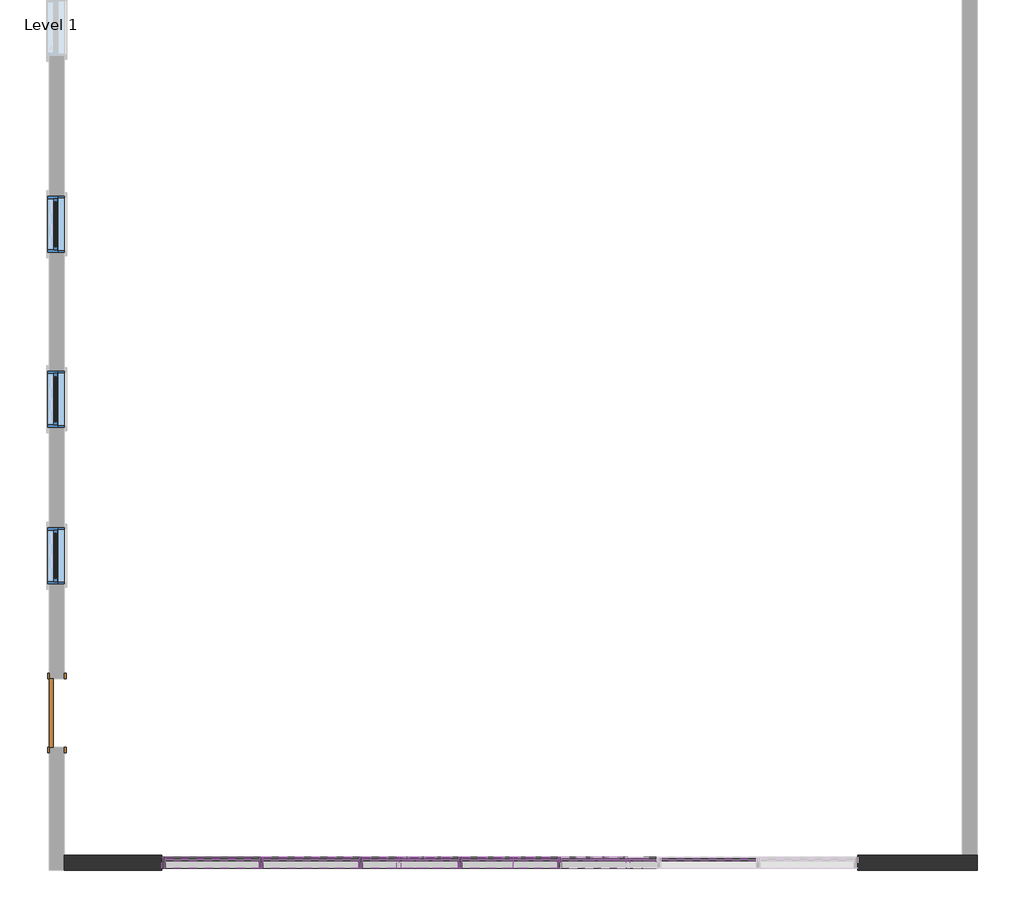
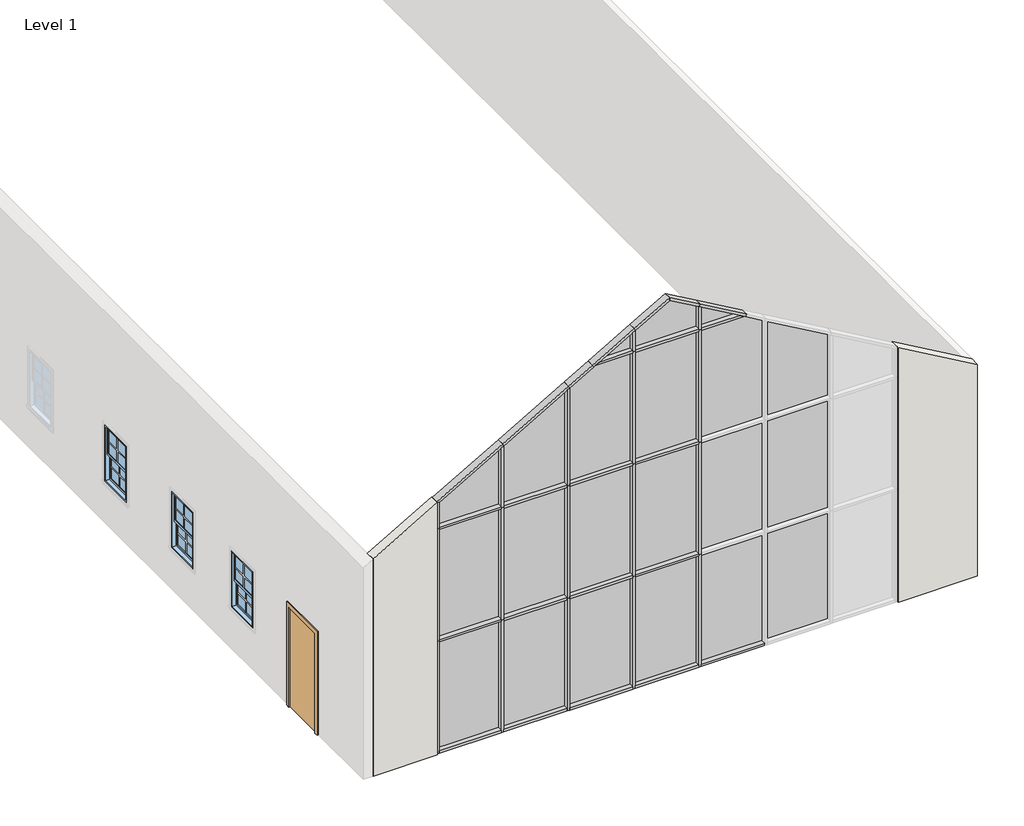
# One storey, part 1 of 2: 40 members, 21 plates, 3 windows, 1 door, 1 wall.
"""IFC4 building model written with IfcOpenShell, lengths in millimetres."""

import ifcopenshell
import ifcopenshell.guid

model = None  # the IFC model being written
_history = None  # IfcOwnerHistory: only IFC2X3 demands one
_inside = {}  # id of a spatial element -> (the spatial element, [elements in it])
_under = {}  # id of a project, library or spatial element -> (it, [spatial elements below it])
_declared = {}  # id of a project -> (the project, [libraries it declares])
_typed = {}  # id of a type object -> (the type object, [elements of that type])
_made_of = {}  # id of a material, layer set ... -> (it, [elements and type objects made of it])


def new_model(schema):
    """Start an empty IFC model of exactly this schema.

    Asked for "IFC4X3", IfcOpenShell would pick the latest addendum, in which some entities
    have other attributes; the version numbers below select the first issue.
    IFC2X3 requires an IfcOwnerHistory on every rooted entity: one is made here for all.
    """
    global model, _history
    if schema == "IFC4X3":
        model = ifcopenshell.file(schema_version=(4, 3, 0, 0))
    else:
        model = ifcopenshell.file(schema=schema)
    _inside.clear()
    _under.clear()
    _declared.clear()
    _typed.clear()
    _made_of.clear()
    _history = None
    if model.schema == "IFC2X3":
        org = make("IfcOrganization", Name="unknown")
        user = make(
            "IfcPersonAndOrganization",
            ThePerson=make("IfcPerson", FamilyName="unknown"),
            TheOrganization=org,
        )
        app = make(
            "IfcApplication",
            ApplicationDeveloper=org,
            Version="unknown",
            ApplicationFullName="unknown",
            ApplicationIdentifier="unknown",
        )
        _history = make(
            "IfcOwnerHistory",
            OwningUser=user,
            OwningApplication=app,
            ChangeAction="ADDED",
            CreationDate=0,
        )
    return model


def make(cls, **values):
    """One entity of the class cls with the attributes given. An attribute that is None is left unset."""
    return model.create_entity(
        cls, **{name: value for name, value in values.items() if value is not None}
    )


def rooted(cls, **values):
    """An entity with a GlobalId (a new one), such as an element, a storey or a relation."""
    return make(cls, GlobalId=ifcopenshell.guid.new(), OwnerHistory=_history, **values)


def si_unit(unit_type, name, prefix=None):
    """IfcSIUnit, for example si_unit("LENGTHUNIT", "METRE", prefix="MILLI")."""
    return make("IfcSIUnit", UnitType=unit_type, Prefix=prefix, Name=name)


def assignment(units):
    """IfcUnitAssignment: the units of a project."""
    return None if units is None else make("IfcUnitAssignment", Units=units)


def point(xyz):
    """IfcCartesianPoint."""
    return None if xyz is None else make("IfcCartesianPoint", Coordinates=xyz)


def direction(xyz):
    """IfcDirection."""
    return None if xyz is None else make("IfcDirection", DirectionRatios=xyz)


def frame(location, z_axis=None, x_axis=None):
    """IfcAxis2Placement3D, a coordinate frame: its origin and axes. An axis left out is left unset."""
    return make(
        "IfcAxis2Placement3D",
        Location=point(location),
        Axis=direction(z_axis),
        RefDirection=direction(x_axis),
    )


def origin():
    """The frame at (0, 0, 0) with its axes left unset."""
    return frame((0.0, 0.0, 0.0))


def origin_with_axes():
    """The frame at (0, 0, 0) with the z axis (0, 0, 1) and the x axis (1, 0, 0) written out."""
    return frame((0.0, 0.0, 0.0), z_axis=(0.0, 0.0, 1.0), x_axis=(1.0, 0.0, 0.0))


def place(relative_to, where):
    """IfcLocalPlacement: puts the frame where relative to a parent placement (None: the world)."""
    return make(
        "IfcLocalPlacement", PlacementRelTo=relative_to, RelativePlacement=where
    )


def context(
    kind, dimensions, precision=None, world=None, true_north=None, identifier=None
):
    """IfcGeometricRepresentationContext, for example the 3D "Model" context."""
    return make(
        "IfcGeometricRepresentationContext",
        ContextIdentifier=identifier,
        ContextType=kind,
        CoordinateSpaceDimension=dimensions,
        Precision=precision,
        WorldCoordinateSystem=world,
        TrueNorth=true_north,
    )


def project(units=None, contexts=None):
    """IfcProject with its units and contexts."""
    return rooted(
        "IfcProject",
        Name="project",
        RepresentationContexts=contexts,
        UnitsInContext=assignment(units),
    )


def spatial(cls, under=None, at=None, **own):
    """A site, building, storey or space (cls), placed at a placement, below another one or the project."""
    s = rooted(cls, ObjectPlacement=at, **own)
    if under is not None:
        _under.setdefault(under.id(), (under, []))[1].append(s)
    return s


def polyline(points):
    """IfcPolyline through the points."""
    return make("IfcPolyline", Points=[point(p) for p in points])


def outline(outer, holes=None, kind="AREA"):
    """IfcArbitraryClosedProfileDef: a profile drawn as a closed curve; with holes, ...WithVoids."""
    if holes is None:
        return make("IfcArbitraryClosedProfileDef", ProfileType=kind, OuterCurve=outer)
    return make(
        "IfcArbitraryProfileDefWithVoids",
        ProfileType=kind,
        OuterCurve=outer,
        InnerCurves=holes,
    )


def extrude(swept, where, along, depth):
    """IfcExtrudedAreaSolid: the profile swept, set in the frame where, extruded along a direction by depth."""
    return make(
        "IfcExtrudedAreaSolid",
        SweptArea=swept,
        Position=where,
        ExtrudedDirection=direction(along),
        Depth=depth,
    )


def faces_of(points, faces, orient=None, outer=None):
    """IfcFace entities. A face is a list of loops; a loop is a list of indices into points, from 0.

    orient and outer hold one flag for each loop. By default every Orientation is true, the
    first loop of a face is its IfcFaceOuterBound and the others are IfcFaceBound.
    """
    made = []
    for i, loops in enumerate(faces):
        bounds = []
        for j, loop in enumerate(loops):
            is_outer = j == 0 if outer is None else outer[i][j]
            bounds.append(
                make(
                    "IfcFaceOuterBound" if is_outer else "IfcFaceBound",
                    Bound=make("IfcPolyLoop", Polygon=[points[k] for k in loop]),
                    Orientation=True if orient is None else orient[i][j],
                )
            )
        made.append(make("IfcFace", Bounds=bounds))
    return made


def faceted_brep(points, faces, orient=None, outer=None, voids=None):
    """IfcFacetedBrep: a solid bounded by flat faces; with voids (closed shells), ...WithVoids."""
    shared = [point(p) for p in points]
    hull = make("IfcClosedShell", CfsFaces=faces_of(shared, faces, orient, outer))
    if voids is None:
        return make("IfcFacetedBrep", Outer=hull)
    return make(
        "IfcFacetedBrepWithVoids",
        Outer=hull,
        Voids=[
            make(cls, CfsFaces=faces_of(shared, fs, o, b)) for cls, fs, o, b in voids
        ],
    )


def shape(context_of_items, identifier, shape_type, items):
    """IfcShapeRepresentation: the items that make up one representation, for example the "Body"."""
    return make(
        "IfcShapeRepresentation",
        ContextOfItems=context_of_items,
        RepresentationIdentifier=identifier,
        RepresentationType=shape_type,
        Items=items,
    )


def source(mapping_origin, context_of_items, identifier, shape_type, items):
    """IfcRepresentationMap: a shape defined once, which mapped items show again and again."""
    return make(
        "IfcRepresentationMap",
        MappingOrigin=mapping_origin,
        MappedRepresentation=shape(context_of_items, identifier, shape_type, items),
    )


def transform(
    local_origin,
    x_axis=None,
    y_axis=None,
    z_axis=None,
    scale=None,
    scale2=None,
    scale3=None,
    uniform=True,
):
    """IfcCartesianTransformationOperator3D, or its non-uniform kind. x_axis, y_axis, z_axis: its Axis1, 2, 3."""
    if uniform:
        return make(
            "IfcCartesianTransformationOperator3D",
            Axis1=direction(x_axis),
            Axis2=direction(y_axis),
            LocalOrigin=point(local_origin),
            Scale=scale,
            Axis3=direction(z_axis),
        )
    return make(
        "IfcCartesianTransformationOperator3DnonUniform",
        Axis1=direction(x_axis),
        Axis2=direction(y_axis),
        LocalOrigin=point(local_origin),
        Scale=scale,
        Axis3=direction(z_axis),
        Scale2=scale2,
        Scale3=scale3,
    )


def mapped(mapping_source, mapping_target):
    """IfcMappedItem: shows the shape of a source again, moved by a transform."""
    return make(
        "IfcMappedItem", MappingSource=mapping_source, MappingTarget=mapping_target
    )


def made_of(thing, what):
    """Note that an element or type object is made of a material, layer set ...; save() writes the relation."""
    if what is not None:
        _made_of.setdefault(what.id(), (what, []))[1].append(thing)
    return thing


def element(
    cls,
    number,
    at=None,
    inside=None,
    cuts=None,
    type_object=None,
    material=None,
    context=None,
    identifier="Body",
    shape_type=None,
    held_by="IfcProductDefinitionShape",
    body=None,
    shapes=None,
    **own,
):
    """One element of the class cls, such as IfcWall. Its Tag is "e" and its number.

    at: its placement. inside: the storey or other place that contains it. cuts: it is an
    opening in that element (IfcRelVoidsElement). A single representation is given by context,
    identifier, shape_type and body (its items); several are given by shapes. held_by: the class
    of the entity that holds the representations. save() writes the other relations.
    """
    e = rooted(cls, Tag="e%d" % number, ObjectPlacement=at, **own)
    if body is not None:
        shapes = [shape(context, identifier, shape_type, body)]
    if shapes is not None:
        e.Representation = make(held_by, Representations=shapes)
    if inside is not None:
        _inside.setdefault(inside.id(), (inside, []))[1].append(e)
    if cuts is not None:
        rooted(
            "IfcRelVoidsElement", RelatingBuildingElement=cuts, RelatedOpeningElement=e
        )
    if type_object is not None:
        _typed.setdefault(type_object.id(), (type_object, []))[1].append(e)
    return made_of(e, material)


def aggregate(whole, parts):
    """IfcRelAggregates: a whole, such as a stair, and the parts it consists of."""
    return rooted("IfcRelAggregates", RelatingObject=whole, RelatedObjects=parts)


def save(model, path):
    """Write the relations noted so far, then the file.

    IfcRelAggregates (storeys below a building ...), IfcRelContainedInSpatialStructure (elements
    in a storey), IfcRelDefinesByType, IfcRelAssociatesMaterial and IfcRelDeclares: one each for
    every whole, place, type object, material and project.
    """
    for whole, parts in _under.values():
        aggregate(whole, parts)
    for where, things in _inside.values():
        rooted(
            "IfcRelContainedInSpatialStructure",
            RelatedElements=things,
            RelatingStructure=where,
        )
    for kind, things in _typed.values():
        rooted("IfcRelDefinesByType", RelatedObjects=things, RelatingType=kind)
    for what, things in _made_of.values():
        rooted("IfcRelAssociatesMaterial", RelatedObjects=things, RelatingMaterial=what)
    for by, libraries in _declared.values():
        rooted("IfcRelDeclares", RelatingContext=by, RelatedDefinitions=libraries)
    model.write(path)


def m_single_flush_0915_x_2134mm_6a9e8738(model_context):
    return source(origin(), model_context, "Body", "SweptSolid", [
        extrude(outline(polyline([(2210.0, -533.5), (0.0, -533.5), (0.0, -457.5), (2134.0, -457.5), (2134.0, 457.5), (0.0, 457.5), (0.0, 533.5), (2210.0, 533.5), (2210.0, -533.5)])), frame((0.0, 100.0, 0.0), z_axis=(0.0, 1.0, 0.0), x_axis=(0.0, 0.0, 1.0)), (0.0, 0.0, 1.0), 25.0),
        extrude(outline(polyline([(2210.0, 533.5), (2210.0, -533.5), (0.0, -533.5), (0.0, -457.5), (2134.0, -457.5), (2134.0, 457.5), (0.0, 457.5), (0.0, 533.5), (2210.0, 533.5)])), frame((0.0, -125.0, 0.0), z_axis=(0.0, 1.0, 0.0), x_axis=(0.0, 0.0, 1.0)), (0.0, 0.0, 1.0), 25.0),
        extrude(outline(polyline([(457.5, 49.0), (-457.5, 49.0), (-457.5, 100.0), (457.5, 100.0), (457.5, 49.0)])), origin_with_axes(), (0.0, 0.0, 1.0), 2134.0),
    ])


def rectangular_mullion_50mm_x_150mm_302a0cfa(model_context):
    return source(origin(), model_context, "Body", "SweptSolid", [
        extrude(outline(polyline([(0.0, 75.0), (0.0, -75.0), (-50.0, -75.0), (-50.0, 75.0), (0.0, 75.0)])), frame((0.0, 0.0, -1253.5714288), z_axis=(0.0, 0.0, 1.0), x_axis=(1.0, 0.0, 0.0)), (0.0, 0.0, 1.0), 1253.5714288),
    ])


def rectangular_mullion_50mm_x_150mm_11a5ee59(model_context):
    return source(origin(), model_context, "Body", "SweptSolid", [
        extrude(outline(polyline([(0.0, 75.0), (0.0, -75.0), (-50.0, -75.0), (-50.0, 75.0), (0.0, 75.0)])), frame((0.0, 0.0, -1278.5714285), z_axis=(0.0, 0.0, 1.0), x_axis=(1.0, 0.0, 0.0)), (0.0, 0.0, 1.0), 1278.5714285),
    ])


def rectangular_mullion_50mm_x_150mm_46426fc7(model_context):
    return source(origin(), model_context, "Body", "SweptSolid", [
        extrude(outline(polyline([(25.0, 75.0), (25.0, -75.0), (-25.0, -75.0), (-25.0, 75.0), (25.0, 75.0)])), frame((0.0, 0.0, -1253.5714288), z_axis=(0.0, 0.0, 1.0), x_axis=(1.0, 0.0, 0.0)), (0.0, 0.0, 1.0), 1253.5714288),
    ])


def rectangular_mullion_50mm_x_150mm_f38f42f6(model_context):
    return source(origin(), model_context, "Body", "SweptSolid", [
        extrude(outline(polyline([(25.0, 75.0), (25.0, -75.0), (-25.0, -75.0), (-25.0, 75.0), (25.0, 75.0)])), frame((0.0, 0.0, -1278.5714285), z_axis=(0.0, 0.0, 1.0), x_axis=(1.0, 0.0, 0.0)), (0.0, 0.0, 1.0), 1278.5714285),
    ])


def rectangular_mullion_50mm_x_150mm_6225e4e3(model_context):
    return source(origin(), model_context, "Body", "SweptSolid", [
        extrude(outline(polyline([(25.0, 75.0), (25.0, -75.0), (-25.0, -75.0), (-25.0, 75.0), (25.0, 75.0)])), frame((0.0, 0.0, -2400.0), z_axis=(0.0, 0.0, 1.0), x_axis=(1.0, 0.0, 0.0)), (0.0, 0.0, 1.0), 2400.0),
    ])


def rectangular_mullion_50mm_x_150mm_662c37b1(model_context):
    return source(origin(), model_context, "Body", "SweptSolid", [
        extrude(outline(polyline([(0.0, 75.0), (0.0, -75.0), (-50.0, -75.0), (-50.0, 75.0), (0.0, 75.0)])), frame((0.0, 0.0, -2400.0), z_axis=(0.0, 0.0, 1.0), x_axis=(1.0, 0.0, 0.0)), (0.0, 0.0, 1.0), 2400.0),
    ])


def rectangular_mullion_50mm_x_150mm_ac9de802(model_context):
    return source(origin(), model_context, "Body", "SweptSolid", [
        extrude(outline(polyline([(0.0, 25.0), (0.0, -25.0), (-761.4529717, -25.0), (-674.8504313, 25.0), (0.0, 25.0)])), frame((0.0, -75.0, 0.0), z_axis=(0.0, 1.0, 0.0), x_axis=(0.0, 0.0, 1.0)), (0.0, 0.0, 1.0), 150.0),
    ])


def rectangular_mullion_50mm_x_150mm_f9b92fbf(model_context):
    return source(origin(), model_context, "Body", "SweptSolid", [
        extrude(outline(polyline([(-143.3012702, 25.0), (-56.6987298, -25.0), (-918.1517015, -25.0), (-918.1517015, 25.0), (-143.3012702, 25.0)])), frame((0.0, -75.0, 0.0), z_axis=(0.0, 1.0, 0.0), x_axis=(0.0, 0.0, 1.0)), (0.0, 0.0, 1.0), 150.0),
    ])


def rectangular_mullion_50mm_x_150mm_ea3fe943(model_context):
    return source(origin(), model_context, "Body", "SweptSolid", [
        extrude(outline(polyline([(0.0, 25.0), (0.0, -25.0), (-1280.5229345, -25.0), (-1309.3904479, 25.0), (0.0, 25.0)])), frame((0.0, -75.0, 0.0), z_axis=(0.0, 1.0, 0.0), x_axis=(0.0, 0.0, 1.0)), (0.0, 0.0, 1.0), 150.0),
    ])


def rectangular_mullion_50mm_x_150mm_5913aded(model_context):
    return source(origin(), model_context, "Body", "SweptSolid", [
        extrude(outline(polyline([(0.0, 25.0), (0.0, -25.0), (-2047.5740063, -25.0), (-2076.4415198, 25.0), (0.0, 25.0)])), frame((0.0, -75.0, 0.0), z_axis=(0.0, 1.0, 0.0), x_axis=(0.0, 0.0, 1.0)), (0.0, 0.0, 1.0), 150.0),
    ])


def rectangular_mullion_50mm_x_150mm_8d818d6c(model_context):
    return source(origin(), model_context, "Body", "SweptSolid", [
        extrude(outline(polyline([(0.0, 25.0), (0.0, -25.0), (-414.6250782, -25.0), (-443.4925917, 25.0), (0.0, 25.0)])), frame((0.0, -75.0, 0.0), z_axis=(0.0, 1.0, 0.0), x_axis=(0.0, 0.0, 1.0)), (0.0, 0.0, 1.0), 150.0),
    ])


def rectangular_mullion_50mm_x_150mm_d4c3fc6e(model_context):
    return source(origin(), model_context, "Body", "SweptSolid", [
        extrude(outline(polyline([(0.0, 25.0), (0.0, -25.0), (-501.2276186, -25.0), (-472.3601051, 25.0), (0.0, 25.0)])), frame((0.0, -75.0, 0.0), z_axis=(0.0, 1.0, 0.0), x_axis=(0.0, 0.0, 1.0)), (0.0, 0.0, 1.0), 150.0),
    ])


def rectangular_mullion_50mm_x_150mm_892e7b11(model_context):
    return source(origin(), model_context, "Body", "SweptSolid", [
        extrude(outline(polyline([(0.0, 0.0), (-28.8675135, -50.0), (-824.7860988, -50.0), (-824.7860988, 0.0), (0.0, 0.0)])), frame((0.0, -75.0, 0.0), z_axis=(0.0, 1.0, 0.0), x_axis=(0.0, 0.0, 1.0)), (0.0, 0.0, 1.0), 150.0),
    ])


def rectangular_mullion_50mm_x_150mm_ed641c16(model_context):
    return source(origin(), model_context, "Body", "SweptSolid", [
        extrude(outline(polyline([(0.0, 0.0), (0.0, -50.0), (-1505.2346306, -50.0), (-1534.1021441, 0.0), (0.0, 0.0)])), frame((0.0, -75.0, 0.0), z_axis=(0.0, 1.0, 0.0), x_axis=(0.0, 0.0, 1.0)), (0.0, 0.0, 1.0), 150.0),
    ])


def rectangular_mullion_50mm_x_150mm_95afd124(model_context):
    return source(origin(), model_context, "Body", "SweptSolid", [
        extrude(outline(polyline([(0.0, 75.0), (0.0, -75.0), (-50.0, -75.0), (-50.0, 75.0), (0.0, 75.0)])), frame((0.0, 0.0, -1534.1021437), z_axis=(0.0, 0.0, 1.0), x_axis=(1.0, 0.0, 0.0)), (0.0, 0.0, 1.0), 1534.1021437),
    ])


def rectangular_mullion_50mm_x_150mm_20c262b5(model_context):
    return source(origin(), model_context, "Body", "SweptSolid", [
        extrude(outline(polyline([(0.0, 75.0), (0.0, -75.0), (-50.0, -75.0), (-50.0, 75.0), (0.0, 75.0)])), frame((0.0, 0.0, -973.5877237), z_axis=(0.0, 0.0, 1.0), x_axis=(1.0, 0.0, 0.0)), (0.0, 0.0, 1.0), 973.5877237),
    ])


def rectangular_mullion_50mm_x_150mm_c61ed2eb(model_context):
    return source(origin(), model_context, "Body", "SweptSolid", [
        extrude(outline(polyline([(0.0, 0.0), (0.0, -50.0), (-680.4485315, -50.0), (-709.316045, 0.0), (0.0, 0.0)])), frame((0.0, -75.0, 0.0), z_axis=(0.0, 1.0, 0.0), x_axis=(0.0, 0.0, 1.0)), (0.0, 0.0, 1.0), 150.0),
    ])


def rectangular_mullion_50mm_x_150mm_579c010a(model_context):
    return source(origin(), model_context, "Body", "SweptSolid", [
        extrude(outline(polyline([(0.0, 75.0), (0.0, -75.0), (-50.0, -75.0), (-50.0, 75.0), (0.0, 75.0)])), frame((0.0, 0.0, -560.51442), z_axis=(0.0, 0.0, 1.0), x_axis=(1.0, 0.0, 0.0)), (0.0, 0.0, 1.0), 560.51442),
    ])


def rectangular_mullion_50mm_x_150mm_be4dfc7d(model_context):
    return source(origin(), model_context, "Body", "SweptSolid", [
        extrude(outline(polyline([(0.0, 75.0), (0.0, -75.0), (-50.0, -75.0), (-50.0, 75.0), (0.0, 75.0)])), frame((0.0, 0.0, -1089.0577775), z_axis=(0.0, 0.0, 1.0), x_axis=(1.0, 0.0, 0.0)), (0.0, 0.0, 1.0), 1089.0577775),
    ])


def rectangular_mullion_50mm_x_150mm_450ea858(model_context):
    return source(origin(), model_context, "Body", "SweptSolid", [
        extrude(outline(polyline([(0.0, 0.0), (-28.8675135, -50.0), (-585.6406461, -50.0), (-585.6406461, 0.0), (0.0, 0.0)])), frame((0.0, -75.0, 0.0), z_axis=(0.0, 1.0, 0.0), x_axis=(0.0, 0.0, 1.0)), (0.0, 0.0, 1.0), 150.0),
    ])


def system_panel_glazed_b60b372a(model_context):
    return source(origin(), model_context, "Body", "SweptSolid", [
        extrude(outline(polyline([(626.7857144, 24.5), (-626.7857144, 24.5), (-626.7857144, 49.5), (626.7857144, 49.5), (626.7857144, 24.5)])), origin_with_axes(), (0.0, 0.0, 1.0), 2325.0),
    ])


def system_panel_glazed_fd68b2ce(model_context):
    return source(origin(), model_context, "Body", "SweptSolid", [
        extrude(outline(polyline([(639.2857142, 24.5), (-639.2857142, 24.5), (-639.2857142, 49.5), (639.2857142, 49.5), (639.2857142, 24.5)])), origin_with_axes(), (0.0, 0.0, 1.0), 2325.0),
    ])


def system_panel_glazed_eec4e8b3(model_context):
    return source(origin(), model_context, "Body", "SweptSolid", [
        extrude(outline(polyline([(626.7857144, 24.5), (-626.7857144, 24.5), (-626.7857144, 49.5), (626.7857144, 49.5), (626.7857144, 24.5)])), origin_with_axes(), (0.0, 0.0, 1.0), 2350.0),
    ])


def system_panel_glazed_5b896d3e(model_context):
    return source(origin(), model_context, "Body", "SweptSolid", [
        extrude(outline(polyline([(639.2857142, 24.5), (-639.2857142, 24.5), (-639.2857142, 49.5), (639.2857142, 49.5), (639.2857142, 24.5)])), origin_with_axes(), (0.0, 0.0, 1.0), 2350.0),
    ])


def system_panel_glazed_ad7ef3dc(model_context):
    return source(origin(), model_context, "Body", "SweptSolid", [
        extrude(outline(polyline([(0.0, -626.7857144), (0.0, 626.7857144), (1255.5229345, 626.7857144), (531.7731326, -626.7857144), (0.0, -626.7857144)])), frame((0.0, 24.5, 0.0), z_axis=(0.0, 1.0, 0.0), x_axis=(0.0, 0.0, 1.0)), (0.0, 0.0, 1.0), 25.0),
    ])


def system_panel_glazed_d3b5986c(model_context):
    return source(origin(), model_context, "Body", "SweptSolid", [
        extrude(outline(polyline([(0.0, -639.2857142), (0.0, 639.2857142), (2022.5740063, 639.2857142), (1284.3904479, -639.2857142), (0.0, -639.2857142)])), frame((0.0, 24.5, 0.0), z_axis=(0.0, 1.0, 0.0), x_axis=(0.0, 0.0, 1.0)), (0.0, 0.0, 1.0), 25.0),
    ])


def system_panel_glazed_fe074b21(model_context):
    return source(origin(), model_context, "Body", "SweptSolid", [
        extrude(outline(polyline([(0.0, -639.2857142), (0.0, 639.2857142), (2350.0, 639.2857142), (2350.0, -178.8659873), (2331.6987298, -153.8659873), (2051.4415198, -639.2857142), (0.0, -639.2857142)])), frame((0.0, 24.5, 0.0), z_axis=(0.0, 1.0, 0.0), x_axis=(0.0, 0.0, 1.0)), (0.0, 0.0, 1.0), 25.0),
    ])


def system_panel_glazed_2c07ae1a(model_context):
    return source(origin(), model_context, "Body", "SweptSolid", [
        extrude(outline(polyline([(0.0, -639.2857142), (0.0, 639.2857142), (2109.1765467, 639.2857142), (2331.6987298, 253.8659873), (2350.0, 278.8659873), (2350.0, -639.2857142), (0.0, -639.2857142)])), frame((0.0, 24.5, 0.0), z_axis=(0.0, 1.0, 0.0), x_axis=(0.0, 0.0, 1.0)), (0.0, 0.0, 1.0), 25.0),
    ])


def system_panel_glazed_d27e4e3c(model_context):
    return source(origin(), model_context, "Body", "SweptSolid", [
        extrude(outline(polyline([(0.0, -639.2857142), (0.0, 639.2857142), (1342.1254748, 639.2857142), (2080.3090332, -639.2857142), (0.0, -639.2857142)])), frame((0.0, 24.5, 0.0), z_axis=(0.0, 1.0, 0.0), x_axis=(0.0, 0.0, 1.0)), (0.0, 0.0, 1.0), 25.0),
    ])


def system_panel_glazed_4ae31ee8(model_context):
    return source(origin(), model_context, "Body", "SweptSolid", [
        extrude(outline(polyline([(0.0, -337.4252157), (0.0, 337.4252157), (389.6250782, 337.4252157), (0.0, -337.4252157)])), frame((0.0, 24.5, 0.0), z_axis=(0.0, 1.0, 0.0), x_axis=(0.0, 0.0, 1.0)), (0.0, 0.0, 1.0), 25.0),
    ])


def system_panel_glazed_71429794(model_context):
    return source(origin(), model_context, "Body", "SweptSolid", [
        extrude(outline(polyline([(0.0, -639.2857142), (0.0, 639.2857142), (476.2276186, 639.2857142), (816.4518843, 50.0), (418.4925917, -639.2857142), (0.0, -639.2857142)])), frame((0.0, 24.5, 0.0), z_axis=(0.0, 1.0, 0.0), x_axis=(0.0, 0.0, 1.0)), (0.0, 0.0, 1.0), 25.0),
    ])


def system_panel_glazed_7669df95(model_context):
    return source(origin(), model_context, "Body", "SweptSolid", [
        extrude(outline(polyline([(0.0, -387.4252157), (0.0, 387.4252157), (447.3601051, -387.4252157), (0.0, -387.4252157)])), frame((0.0, 24.5, 0.0), z_axis=(0.0, 1.0, 0.0), x_axis=(0.0, 0.0, 1.0)), (0.0, 0.0, 1.0), 25.0),
    ])


def m_window_double_hung_750_x_1200mm_41070976(model_context):
    return source(origin(), model_context, "Body", "SweptSolid", [
        extrude(outline(polyline([(298.8, 30.15), (298.8, 23.8), (-298.8, 23.8), (-298.8, 30.15), (298.8, 30.15)])), frame((0.0, 0.0, 990.6), z_axis=(0.0, 0.0, 1.0), x_axis=(1.0, 0.0, 0.0)), (0.0, 0.0, 1.0), 501.575),
        extrude(outline(polyline([(-298.8, 17.45), (298.8, 17.45), (298.8, 11.1), (-298.8, 11.1), (-298.8, 17.45)])), frame((0.0, 0.0, 990.6), z_axis=(0.0, 0.0, 1.0), x_axis=(1.0, 0.0, 0.0)), (0.0, 0.0, 1.0), 501.575),
        extrude(outline(polyline([(298.8, 74.6), (298.8, 68.25), (-298.8, 68.25), (-298.8, 74.6), (298.8, 74.6)])), frame((0.0, 0.0, 1536.625), z_axis=(0.0, 0.0, 1.0), x_axis=(1.0, 0.0, 0.0)), (0.0, 0.0, 1.0), 501.575),
        extrude(outline(polyline([(-298.8, 61.9), (298.8, 61.9), (298.8, 55.55), (-298.8, 55.55), (-298.8, 61.9)])), frame((0.0, 0.0, 1536.625), z_axis=(0.0, 0.0, 1.0), x_axis=(1.0, 0.0, 0.0)), (0.0, 0.0, 1.0), 501.575),
        extrude(outline(polyline([(1536.625, -343.25), (946.15, -343.25), (946.15, 343.25), (1536.625, 343.25), (1536.625, -343.25)]), holes=[polyline([(1492.175, 298.8), (990.6, 298.8), (990.6, -298.8), (1492.175, -298.8), (1492.175, 298.8)])]), frame((0.0, -1.6, 0.0), z_axis=(0.0, 1.0, 0.0), x_axis=(0.0, 0.0, 1.0)), (0.0, 0.0, 1.0), 44.45),
        extrude(outline(polyline([(2082.65, -343.25), (1492.175, -343.25), (1492.175, 343.25), (2082.65, 343.25), (2082.65, -343.25)]), holes=[polyline([(2038.2, 298.8), (1536.625, 298.8), (1536.625, -298.8), (2038.2, -298.8), (2038.2, 298.8)])]), frame((0.0, 42.85, 0.0), z_axis=(0.0, 1.0, 0.0), x_axis=(0.0, 0.0, 1.0)), (0.0, 0.0, 1.0), 44.45),
        extrude(outline(polyline([(2114.4, -375.0), (914.4, -375.0), (914.4, 375.0), (2114.4, 375.0), (2114.4, -375.0)]), holes=[polyline([(2082.65, 343.25), (946.15, 343.25), (946.15, -343.25), (2082.65, -343.25), (2082.65, 343.25)])]), frame((0.0, -14.3, 0.0), z_axis=(0.0, 1.0, 0.0), x_axis=(0.0, 0.0, 1.0)), (0.0, 0.0, 1.0), 133.35),
        extrude(outline(polyline([(2114.4, 375.0), (2114.4, -375.0), (914.4, -375.0), (914.4, 375.0), (2114.4, 375.0)]), holes=[polyline([(2095.35, 355.95), (933.45, 355.95), (933.45, -355.95), (2095.35, -355.95), (2095.35, 355.95)])]), frame((0.0, -100.0, 0.0), z_axis=(0.0, 1.0, 0.0), x_axis=(0.0, 0.0, 1.0)), (0.0, 0.0, 1.0), 85.7),
    ])


model = new_model("IFC4")

# Units and contexts
model_context = context("Model", 3, world=origin())
ifc_project = project(units=[si_unit("LENGTHUNIT", "METRE", prefix="MILLI")], contexts=[model_context])

# Site, building, storey
site = spatial("IfcSite", under=ifc_project)
building = spatial("IfcBuilding", under=site)
storey = spatial("IfcBuildingStorey", under=building, Name="Level 1", Elevation=0.0)

# Door
placement = place(None, origin())
m_single_flush_0915_x_2134mm_shape = m_single_flush_0915_x_2134mm_6a9e8738(model_context)
element("IfcDoor", 1, ObjectType="M_Single-Flush : 0915 x 2134mm", at=placement, inside=storey, context=model_context, shape_type="MappedRepresentation", body=[
    mapped(m_single_flush_0915_x_2134mm_shape, transform((-6967.834392, -6666.9793434, 0.0), x_axis=(0.0, 1.0, 0.0), y_axis=(-1.0, 0.0, 0.0), z_axis=(0.0, 0.0, 1.0))),
])

# Members
rectangular_mullion_50mm_x_150mm_shape = rectangular_mullion_50mm_x_150mm_302a0cfa(model_context)
element("IfcMember", 2, ObjectType="Rectangular Mullion : 50mm x 150mm", at=placement, inside=storey, context=model_context, shape_type="MappedRepresentation", body=[
    mapped(rectangular_mullion_50mm_x_150mm_shape, transform((-5517.834392, -8666.9793434, 0.0), x_axis=(0.0, 0.0, -1.0), y_axis=(0.0, -1.0, 0.0), z_axis=(-1.0, 0.0, 0.0))),
])
rectangular_mullion_50mm_x_150mm_2_shape = rectangular_mullion_50mm_x_150mm_11a5ee59(model_context)
element("IfcMember", 3, ObjectType="Rectangular Mullion : 50mm x 150mm", at=placement, inside=storey, context=model_context, shape_type="MappedRepresentation", body=[
    mapped(rectangular_mullion_50mm_x_150mm_2_shape, transform((-4214.2629632, -8666.9793434, 0.0), x_axis=(0.0, 0.0, -1.0), y_axis=(0.0, -1.0, 0.0), z_axis=(-1.0, 0.0, 0.0))),
])
element("IfcMember", 4, ObjectType="Rectangular Mullion : 50mm x 150mm", at=placement, inside=storey, context=model_context, shape_type="MappedRepresentation", body=[
    mapped(rectangular_mullion_50mm_x_150mm_2_shape, transform((-2885.6915347, -8666.9793434, 0.0), x_axis=(0.0, 0.0, -1.0), y_axis=(0.0, -1.0, 0.0), z_axis=(-1.0, 0.0, 0.0))),
])
element("IfcMember", 5, ObjectType="Rectangular Mullion : 50mm x 150mm", at=placement, inside=storey, context=model_context, shape_type="MappedRepresentation", body=[
    mapped(rectangular_mullion_50mm_x_150mm_2_shape, transform((-1557.1201062, -8666.9793434, 0.0), x_axis=(0.0, 0.0, -1.0), y_axis=(0.0, -1.0, 0.0), z_axis=(-1.0, 0.0, 0.0))),
])
element("IfcMember", 6, ObjectType="Rectangular Mullion : 50mm x 150mm", at=placement, inside=storey, context=model_context, shape_type="MappedRepresentation", body=[
    mapped(rectangular_mullion_50mm_x_150mm_2_shape, transform((-228.5486777, -8666.9793434, 0.0), x_axis=(0.0, 0.0, -1.0), y_axis=(0.0, -1.0, 0.0), z_axis=(-1.0, 0.0, 0.0))),
])
rectangular_mullion_50mm_x_150mm_3_shape = rectangular_mullion_50mm_x_150mm_46426fc7(model_context)
element("IfcMember", 7, ObjectType="Rectangular Mullion : 50mm x 150mm", at=placement, inside=storey, context=model_context, shape_type="MappedRepresentation", body=[
    mapped(rectangular_mullion_50mm_x_150mm_3_shape, transform((-4264.2629632, -8666.9793434, 2400.0), x_axis=(0.0, 0.0, 1.0), y_axis=(0.0, -1.0, 0.0), z_axis=(1.0, 0.0, 0.0))),
])
element("IfcMember", 8, ObjectType="Rectangular Mullion : 50mm x 150mm", at=placement, inside=storey, context=model_context, shape_type="MappedRepresentation", body=[
    mapped(rectangular_mullion_50mm_x_150mm_3_shape, transform((-4264.2629632, -8666.9793434, 4800.0), x_axis=(0.0, 0.0, 1.0), y_axis=(0.0, -1.0, 0.0), z_axis=(1.0, 0.0, 0.0))),
])
rectangular_mullion_50mm_x_150mm_4_shape = rectangular_mullion_50mm_x_150mm_f38f42f6(model_context)
element("IfcMember", 9, ObjectType="Rectangular Mullion : 50mm x 150mm", at=placement, inside=storey, context=model_context, shape_type="MappedRepresentation", body=[
    mapped(rectangular_mullion_50mm_x_150mm_4_shape, transform((-2935.6915347, -8666.9793434, 2400.0), x_axis=(0.0, 0.0, 1.0), y_axis=(0.0, -1.0, 0.0), z_axis=(1.0, 0.0, 0.0))),
])
element("IfcMember", 10, ObjectType="Rectangular Mullion : 50mm x 150mm", at=placement, inside=storey, context=model_context, shape_type="MappedRepresentation", body=[
    mapped(rectangular_mullion_50mm_x_150mm_4_shape, transform((-1607.1201062, -8666.9793434, 2400.0), x_axis=(0.0, 0.0, 1.0), y_axis=(0.0, -1.0, 0.0), z_axis=(1.0, 0.0, 0.0))),
])
element("IfcMember", 11, ObjectType="Rectangular Mullion : 50mm x 150mm", at=placement, inside=storey, context=model_context, shape_type="MappedRepresentation", body=[
    mapped(rectangular_mullion_50mm_x_150mm_4_shape, transform((-278.5486777, -8666.9793434, 2400.0), x_axis=(0.0, 0.0, 1.0), y_axis=(0.0, -1.0, 0.0), z_axis=(1.0, 0.0, 0.0))),
])
element("IfcMember", 12, ObjectType="Rectangular Mullion : 50mm x 150mm", at=placement, inside=storey, context=model_context, shape_type="MappedRepresentation", body=[
    mapped(rectangular_mullion_50mm_x_150mm_4_shape, transform((-2935.6915347, -8666.9793434, 4800.0), x_axis=(0.0, 0.0, 1.0), y_axis=(0.0, -1.0, 0.0), z_axis=(1.0, 0.0, 0.0))),
])
element("IfcMember", 13, ObjectType="Rectangular Mullion : 50mm x 150mm", at=placement, inside=storey, context=model_context, shape_type="MappedRepresentation", body=[
    mapped(rectangular_mullion_50mm_x_150mm_4_shape, transform((-1607.1201062, -8666.9793434, 4800.0), x_axis=(0.0, 0.0, 1.0), y_axis=(0.0, -1.0, 0.0), z_axis=(1.0, 0.0, 0.0))),
])
element("IfcMember", 14, ObjectType="Rectangular Mullion : 50mm x 150mm", at=placement, inside=storey, context=model_context, shape_type="MappedRepresentation", body=[
    mapped(rectangular_mullion_50mm_x_150mm_4_shape, transform((-278.5486777, -8666.9793434, 4800.0), x_axis=(0.0, 0.0, 1.0), y_axis=(0.0, -1.0, 0.0), z_axis=(1.0, 0.0, 0.0))),
])
element("IfcMember", 15, ObjectType="Rectangular Mullion : 50mm x 150mm", at=placement, inside=storey, context=model_context, shape_type="MappedRepresentation", body=[
    mapped(rectangular_mullion_50mm_x_150mm_4_shape, transform((-278.5486777, -8666.9793434, 7200.0), x_axis=(0.0, 0.0, 1.0), y_axis=(0.0, -1.0, 0.0), z_axis=(1.0, 0.0, 0.0))),
])
rectangular_mullion_50mm_x_150mm_5_shape = rectangular_mullion_50mm_x_150mm_6225e4e3(model_context)
element("IfcMember", 16, ObjectType="Rectangular Mullion : 50mm x 150mm", at=placement, inside=storey, context=model_context, shape_type="MappedRepresentation", body=[
    mapped(rectangular_mullion_50mm_x_150mm_5_shape, transform((-4239.2629632, -8666.9793434, 0.0), x_axis=(1.0, 0.0, 0.0), y_axis=(0.0, -1.0, 0.0), z_axis=(0.0, 0.0, -1.0))),
])
element("IfcMember", 17, ObjectType="Rectangular Mullion : 50mm x 150mm", at=placement, inside=storey, context=model_context, shape_type="MappedRepresentation", body=[
    mapped(rectangular_mullion_50mm_x_150mm_5_shape, transform((-2910.6915347, -8666.9793434, 0.0), x_axis=(1.0, 0.0, 0.0), y_axis=(0.0, -1.0, 0.0), z_axis=(0.0, 0.0, -1.0))),
])
element("IfcMember", 18, ObjectType="Rectangular Mullion : 50mm x 150mm", at=placement, inside=storey, context=model_context, shape_type="MappedRepresentation", body=[
    mapped(rectangular_mullion_50mm_x_150mm_5_shape, transform((-1582.1201062, -8666.9793434, 0.0), x_axis=(1.0, 0.0, 0.0), y_axis=(0.0, -1.0, 0.0), z_axis=(0.0, 0.0, -1.0))),
])
element("IfcMember", 19, ObjectType="Rectangular Mullion : 50mm x 150mm", at=placement, inside=storey, context=model_context, shape_type="MappedRepresentation", body=[
    mapped(rectangular_mullion_50mm_x_150mm_5_shape, transform((-253.5486777, -8666.9793434, 0.0), x_axis=(1.0, 0.0, 0.0), y_axis=(0.0, -1.0, 0.0), z_axis=(0.0, 0.0, -1.0))),
])
element("IfcMember", 20, ObjectType="Rectangular Mullion : 50mm x 150mm", at=placement, inside=storey, context=model_context, shape_type="MappedRepresentation", body=[
    mapped(rectangular_mullion_50mm_x_150mm_5_shape, transform((-4239.2629632, -8666.9793434, 2400.0), x_axis=(1.0, 0.0, 0.0), y_axis=(0.0, -1.0, 0.0), z_axis=(0.0, 0.0, -1.0))),
])
element("IfcMember", 21, ObjectType="Rectangular Mullion : 50mm x 150mm", at=placement, inside=storey, context=model_context, shape_type="MappedRepresentation", body=[
    mapped(rectangular_mullion_50mm_x_150mm_5_shape, transform((-2910.6915347, -8666.9793434, 2400.0), x_axis=(1.0, 0.0, 0.0), y_axis=(0.0, -1.0, 0.0), z_axis=(0.0, 0.0, -1.0))),
])
element("IfcMember", 22, ObjectType="Rectangular Mullion : 50mm x 150mm", at=placement, inside=storey, context=model_context, shape_type="MappedRepresentation", body=[
    mapped(rectangular_mullion_50mm_x_150mm_5_shape, transform((-1582.1201062, -8666.9793434, 2400.0), x_axis=(1.0, 0.0, 0.0), y_axis=(0.0, -1.0, 0.0), z_axis=(0.0, 0.0, -1.0))),
])
element("IfcMember", 23, ObjectType="Rectangular Mullion : 50mm x 150mm", at=placement, inside=storey, context=model_context, shape_type="MappedRepresentation", body=[
    mapped(rectangular_mullion_50mm_x_150mm_5_shape, transform((-253.5486777, -8666.9793434, 2400.0), x_axis=(1.0, 0.0, 0.0), y_axis=(0.0, -1.0, 0.0), z_axis=(0.0, 0.0, -1.0))),
])
element("IfcMember", 24, ObjectType="Rectangular Mullion : 50mm x 150mm", at=placement, inside=storey, context=model_context, shape_type="MappedRepresentation", body=[
    mapped(rectangular_mullion_50mm_x_150mm_5_shape, transform((-1582.1201062, -8666.9793434, 4800.0), x_axis=(1.0, 0.0, 0.0), y_axis=(0.0, -1.0, 0.0), z_axis=(0.0, 0.0, -1.0))),
])
element("IfcMember", 25, ObjectType="Rectangular Mullion : 50mm x 150mm", at=placement, inside=storey, context=model_context, shape_type="MappedRepresentation", body=[
    mapped(rectangular_mullion_50mm_x_150mm_5_shape, transform((-253.5486777, -8666.9793434, 4800.0), x_axis=(1.0, 0.0, 0.0), y_axis=(0.0, -1.0, 0.0), z_axis=(0.0, 0.0, -1.0))),
])
rectangular_mullion_50mm_x_150mm_6_shape = rectangular_mullion_50mm_x_150mm_662c37b1(model_context)
element("IfcMember", 26, ObjectType="Rectangular Mullion : 50mm x 150mm", at=placement, inside=storey, context=model_context, shape_type="MappedRepresentation", body=[
    mapped(rectangular_mullion_50mm_x_150mm_6_shape, transform((-5567.834392, -8666.9793434, 2400.0), x_axis=(-1.0, 0.0, 0.0), y_axis=(0.0, -1.0, 0.0), z_axis=(0.0, 0.0, 1.0))),
])
element("IfcMember", 27, ObjectType="Rectangular Mullion : 50mm x 150mm", at=placement, inside=storey, context=model_context, shape_type="MappedRepresentation", body=[
    mapped(rectangular_mullion_50mm_x_150mm_6_shape, transform((-5567.834392, -8666.9793434, 4800.0), x_axis=(-1.0, 0.0, 0.0), y_axis=(0.0, -1.0, 0.0), z_axis=(0.0, 0.0, 1.0))),
])
rectangular_mullion_50mm_x_150mm_7_shape = rectangular_mullion_50mm_x_150mm_ac9de802(model_context)
element("IfcMember", 28, ObjectType="Rectangular Mullion : 50mm x 150mm", at=placement, inside=storey, context=model_context, shape_type="MappedRepresentation", body=[
    mapped(rectangular_mullion_50mm_x_150mm_7_shape, transform((-1607.1201062, -8666.9793434, 7200.0), x_axis=(0.0, 0.0, 1.0), y_axis=(0.0, -1.0, 0.0), z_axis=(1.0, 0.0, 0.0))),
])
rectangular_mullion_50mm_x_150mm_8_shape = rectangular_mullion_50mm_x_150mm_f9b92fbf(model_context)
element("IfcMember", 29, ObjectType="Rectangular Mullion : 50mm x 150mm", at=placement, inside=storey, context=model_context, shape_type="MappedRepresentation", body=[
    mapped(rectangular_mullion_50mm_x_150mm_8_shape, transform((689.6030238, -8666.9793434, 7200.0), x_axis=(0.0, 0.0, 1.0), y_axis=(0.0, -1.0, 0.0), z_axis=(1.0, 0.0, 0.0))),
])
rectangular_mullion_50mm_x_150mm_9_shape = rectangular_mullion_50mm_x_150mm_ea3fe943(model_context)
element("IfcMember", 30, ObjectType="Rectangular Mullion : 50mm x 150mm", at=placement, inside=storey, context=model_context, shape_type="MappedRepresentation", body=[
    mapped(rectangular_mullion_50mm_x_150mm_9_shape, transform((-4239.2629632, -8666.9793434, 4800.0), x_axis=(1.0, 0.0, 0.0), y_axis=(0.0, -1.0, 0.0), z_axis=(0.0, 0.0, -1.0))),
])
rectangular_mullion_50mm_x_150mm_10_shape = rectangular_mullion_50mm_x_150mm_5913aded(model_context)
element("IfcMember", 31, ObjectType="Rectangular Mullion : 50mm x 150mm", at=placement, inside=storey, context=model_context, shape_type="MappedRepresentation", body=[
    mapped(rectangular_mullion_50mm_x_150mm_10_shape, transform((-2910.6915347, -8666.9793434, 4800.0), x_axis=(1.0, 0.0, 0.0), y_axis=(0.0, -1.0, 0.0), z_axis=(0.0, 0.0, -1.0))),
])
rectangular_mullion_50mm_x_150mm_11_shape = rectangular_mullion_50mm_x_150mm_8d818d6c(model_context)
element("IfcMember", 32, ObjectType="Rectangular Mullion : 50mm x 150mm", at=placement, inside=storey, context=model_context, shape_type="MappedRepresentation", body=[
    mapped(rectangular_mullion_50mm_x_150mm_11_shape, transform((-1582.1201062, -8666.9793434, 7200.0), x_axis=(1.0, 0.0, 0.0), y_axis=(0.0, -1.0, 0.0), z_axis=(0.0, 0.0, -1.0))),
])
rectangular_mullion_50mm_x_150mm_12_shape = rectangular_mullion_50mm_x_150mm_d4c3fc6e(model_context)
element("IfcMember", 33, ObjectType="Rectangular Mullion : 50mm x 150mm", at=placement, inside=storey, context=model_context, shape_type="MappedRepresentation", body=[
    mapped(rectangular_mullion_50mm_x_150mm_12_shape, transform((-253.5486777, -8666.9793434, 7200.0), x_axis=(1.0, 0.0, 0.0), y_axis=(0.0, -1.0, 0.0), z_axis=(0.0, 0.0, -1.0))),
])
rectangular_mullion_50mm_x_150mm_13_shape = rectangular_mullion_50mm_x_150mm_892e7b11(model_context)
element("IfcMember", 34, ObjectType="Rectangular Mullion : 50mm x 150mm", at=placement, inside=storey, context=model_context, shape_type="MappedRepresentation", body=[
    mapped(rectangular_mullion_50mm_x_150mm_13_shape, transform((-867.834392, -8666.9793434, 8099.1869112), x_axis=(-0.5000000000000014, 0.0, 0.8660254037844379), y_axis=(0.0, -1.0, 0.0), z_axis=(0.8660254037844379, 0.0, 0.5000000000000014))),
])
rectangular_mullion_50mm_x_150mm_14_shape = rectangular_mullion_50mm_x_150mm_ed641c16(model_context)
element("IfcMember", 35, ObjectType="Rectangular Mullion : 50mm x 150mm", at=placement, inside=storey, context=model_context, shape_type="MappedRepresentation", body=[
    mapped(rectangular_mullion_50mm_x_150mm_14_shape, transform((-4239.2629632, -8666.9793434, 6152.6917181), x_axis=(-0.5000000000000007, 0.0, 0.8660254037844384), y_axis=(0.0, -1.0, 0.0), z_axis=(0.8660254037844383, 0.0, 0.5000000000000006))),
])
rectangular_mullion_50mm_x_150mm_15_shape = rectangular_mullion_50mm_x_150mm_95afd124(model_context)
element("IfcMember", 36, ObjectType="Rectangular Mullion : 50mm x 150mm", at=placement, inside=storey, context=model_context, shape_type="MappedRepresentation", body=[
    mapped(rectangular_mullion_50mm_x_150mm_15_shape, transform((-2910.6915347, -8666.9793434, 6919.74279), x_axis=(-0.5000000000000001, 0.0, 0.8660254037844387), y_axis=(0.0, -1.0, 0.0), z_axis=(0.8660254037844387, 0.0, 0.5000000000000001))),
])
rectangular_mullion_50mm_x_150mm_16_shape = rectangular_mullion_50mm_x_150mm_20c262b5(model_context)
element("IfcMember", 37, ObjectType="Rectangular Mullion : 50mm x 150mm", at=placement, inside=storey, context=model_context, shape_type="MappedRepresentation", body=[
    mapped(rectangular_mullion_50mm_x_150mm_16_shape, transform((-1582.1201062, -8666.9793434, 7686.7938619), x_axis=(-0.5000000000000003, 0.0, 0.8660254037844385), y_axis=(0.0, -1.0, 0.0), z_axis=(0.8660254037844385, 0.0, 0.5000000000000003))),
])
rectangular_mullion_50mm_x_150mm_17_shape = rectangular_mullion_50mm_x_150mm_c61ed2eb(model_context)
element("IfcMember", 38, ObjectType="Rectangular Mullion : 50mm x 150mm", at=placement, inside=storey, context=model_context, shape_type="MappedRepresentation", body=[
    mapped(rectangular_mullion_50mm_x_150mm_17_shape, transform((-253.5486777, -8666.9793434, 7744.5288888), x_axis=(0.5000000000000002, 0.0, 0.8660254037844386), y_axis=(0.0, -1.0, 0.0), z_axis=(0.8660254037844386, 0.0, -0.5000000000000002))),
])
rectangular_mullion_50mm_x_150mm_18_shape = rectangular_mullion_50mm_x_150mm_579c010a(model_context)
element("IfcMember", 39, ObjectType="Rectangular Mullion : 50mm x 150mm", at=placement, inside=storey, context=model_context, shape_type="MappedRepresentation", body=[
    mapped(rectangular_mullion_50mm_x_150mm_18_shape, transform((-2425.2718077, -8666.9793434, 7200.0), x_axis=(-0.5000000000000004, 0.0, 0.8660254037844385), y_axis=(0.0, -1.0, 0.0), z_axis=(0.8660254037844385, 0.0, 0.5000000000000004))),
])
rectangular_mullion_50mm_x_150mm_19_shape = rectangular_mullion_50mm_x_150mm_be4dfc7d(model_context)
element("IfcMember", 40, ObjectType="Rectangular Mullion : 50mm x 150mm", at=placement, inside=storey, context=model_context, shape_type="MappedRepresentation", body=[
    mapped(rectangular_mullion_50mm_x_150mm_19_shape, transform((689.6030238, -8666.9793434, 7200.0), x_axis=(0.5000000000000007, 0.0, 0.8660254037844383), y_axis=(0.0, -1.0, 0.0), z_axis=(0.8660254037844383, 0.0, -0.5000000000000007))),
])
rectangular_mullion_50mm_x_150mm_20_shape = rectangular_mullion_50mm_x_150mm_450ea858(model_context)
element("IfcMember", 41, ObjectType="Rectangular Mullion : 50mm x 150mm", at=placement, inside=storey, context=model_context, shape_type="MappedRepresentation", body=[
    mapped(rectangular_mullion_50mm_x_150mm_20_shape, transform((-5567.834392, -8666.9793434, 5385.6406461), x_axis=(-1.0, 0.0, 0.0), y_axis=(0.0, -1.0, 0.0), z_axis=(0.0, 0.0, 1.0))),
])

# Plates
system_panel_glazed_shape = system_panel_glazed_b60b372a(model_context)
element("IfcPlate", 42, ObjectType="System Panel : Glazed", at=placement, inside=storey, context=model_context, shape_type="MappedRepresentation", body=[
    mapped(system_panel_glazed_shape, transform((-4891.0486776, -8666.9793434, 50.0), x_axis=(1.0, 0.0, 0.0), y_axis=(0.0, 1.0, 0.0), z_axis=(0.0, 0.0, 1.0))),
])
system_panel_glazed_2_shape = system_panel_glazed_fd68b2ce(model_context)
element("IfcPlate", 43, ObjectType="System Panel : Glazed", at=placement, inside=storey, context=model_context, shape_type="MappedRepresentation", body=[
    mapped(system_panel_glazed_2_shape, transform((-3574.9772489, -8666.9793434, 50.0), x_axis=(1.0, 0.0, 0.0), y_axis=(0.0, 1.0, 0.0), z_axis=(0.0, 0.0, 1.0))),
])
element("IfcPlate", 44, ObjectType="System Panel : Glazed", at=placement, inside=storey, context=model_context, shape_type="MappedRepresentation", body=[
    mapped(system_panel_glazed_2_shape, transform((-2246.4058204, -8666.9793434, 50.0), x_axis=(1.0, 0.0, 0.0), y_axis=(0.0, 1.0, 0.0), z_axis=(0.0, 0.0, 1.0))),
])
element("IfcPlate", 45, ObjectType="System Panel : Glazed", at=placement, inside=storey, context=model_context, shape_type="MappedRepresentation", body=[
    mapped(system_panel_glazed_2_shape, transform((-917.834392, -8666.9793434, 50.0), x_axis=(1.0, 0.0, 0.0), y_axis=(0.0, 1.0, 0.0), z_axis=(0.0, 0.0, 1.0))),
])
element("IfcPlate", 46, ObjectType="System Panel : Glazed", at=placement, inside=storey, context=model_context, shape_type="MappedRepresentation", body=[
    mapped(system_panel_glazed_2_shape, transform((410.7370365, -8666.9793434, 50.0), x_axis=(1.0, 0.0, 0.0), y_axis=(0.0, 1.0, 0.0), z_axis=(0.0, 0.0, 1.0))),
])
element("IfcPlate", 47, ObjectType="System Panel : Glazed", at=placement, inside=storey, context=model_context, shape_type="MappedRepresentation", body=[
    mapped(system_panel_glazed_2_shape, transform((1739.308465, -8666.9793434, 50.0), x_axis=(1.0, 0.0, 0.0), y_axis=(0.0, 1.0, 0.0), z_axis=(0.0, 0.0, 1.0))),
])
system_panel_glazed_3_shape = system_panel_glazed_eec4e8b3(model_context)
element("IfcPlate", 48, ObjectType="System Panel : Glazed", at=placement, inside=storey, context=model_context, shape_type="MappedRepresentation", body=[
    mapped(system_panel_glazed_3_shape, transform((-4891.0486776, -8666.9793434, 2425.0), x_axis=(1.0, 0.0, 0.0), y_axis=(0.0, 1.0, 0.0), z_axis=(0.0, 0.0, 1.0))),
])
system_panel_glazed_4_shape = system_panel_glazed_5b896d3e(model_context)
element("IfcPlate", 49, ObjectType="System Panel : Glazed", at=placement, inside=storey, context=model_context, shape_type="MappedRepresentation", body=[
    mapped(system_panel_glazed_4_shape, transform((-3574.9772489, -8666.9793434, 2425.0), x_axis=(1.0, 0.0, 0.0), y_axis=(0.0, 1.0, 0.0), z_axis=(0.0, 0.0, 1.0))),
])
element("IfcPlate", 50, ObjectType="System Panel : Glazed", at=placement, inside=storey, context=model_context, shape_type="MappedRepresentation", body=[
    mapped(system_panel_glazed_4_shape, transform((-2246.4058204, -8666.9793434, 2425.0), x_axis=(1.0, 0.0, 0.0), y_axis=(0.0, 1.0, 0.0), z_axis=(0.0, 0.0, 1.0))),
])
element("IfcPlate", 51, ObjectType="System Panel : Glazed", at=placement, inside=storey, context=model_context, shape_type="MappedRepresentation", body=[
    mapped(system_panel_glazed_4_shape, transform((-917.834392, -8666.9793434, 2425.0), x_axis=(1.0, 0.0, 0.0), y_axis=(0.0, 1.0, 0.0), z_axis=(0.0, 0.0, 1.0))),
])
element("IfcPlate", 52, ObjectType="System Panel : Glazed", at=placement, inside=storey, context=model_context, shape_type="MappedRepresentation", body=[
    mapped(system_panel_glazed_4_shape, transform((410.7370365, -8666.9793434, 2425.0), x_axis=(1.0, 0.0, 0.0), y_axis=(0.0, 1.0, 0.0), z_axis=(0.0, 0.0, 1.0))),
])
element("IfcPlate", 53, ObjectType="System Panel : Glazed", at=placement, inside=storey, context=model_context, shape_type="MappedRepresentation", body=[
    mapped(system_panel_glazed_4_shape, transform((1739.308465, -8666.9793434, 2425.0), x_axis=(1.0, 0.0, 0.0), y_axis=(0.0, 1.0, 0.0), z_axis=(0.0, 0.0, 1.0))),
])
element("IfcPlate", 54, ObjectType="System Panel : Glazed", at=placement, inside=storey, context=model_context, shape_type="MappedRepresentation", body=[
    mapped(system_panel_glazed_4_shape, transform((-917.834392, -8666.9793434, 4825.0), x_axis=(1.0, 0.0, 0.0), y_axis=(0.0, 1.0, 0.0), z_axis=(0.0, 0.0, 1.0))),
])
system_panel_glazed_5_shape = system_panel_glazed_ad7ef3dc(model_context)
element("IfcPlate", 55, ObjectType="System Panel : Glazed", at=placement, inside=storey, context=model_context, shape_type="MappedRepresentation", body=[
    mapped(system_panel_glazed_5_shape, transform((-4891.0486776, -8666.9793434, 4825.0), x_axis=(1.0, 0.0, 0.0), y_axis=(0.0, 1.0, 0.0), z_axis=(0.0, 0.0, 1.0))),
])
system_panel_glazed_6_shape = system_panel_glazed_d3b5986c(model_context)
element("IfcPlate", 56, ObjectType="System Panel : Glazed", at=placement, inside=storey, context=model_context, shape_type="MappedRepresentation", body=[
    mapped(system_panel_glazed_6_shape, transform((-3574.9772489, -8666.9793434, 4825.0), x_axis=(1.0, 0.0, 0.0), y_axis=(0.0, 1.0, 0.0), z_axis=(0.0, 0.0, 1.0))),
])
system_panel_glazed_7_shape = system_panel_glazed_fe074b21(model_context)
element("IfcPlate", 57, ObjectType="System Panel : Glazed", at=placement, inside=storey, context=model_context, shape_type="MappedRepresentation", body=[
    mapped(system_panel_glazed_7_shape, transform((-2246.4058204, -8666.9793434, 4825.0), x_axis=(1.0, 0.0, 0.0), y_axis=(0.0, 1.0, 0.0), z_axis=(0.0, 0.0, 1.0))),
])
system_panel_glazed_8_shape = system_panel_glazed_2c07ae1a(model_context)
element("IfcPlate", 58, ObjectType="System Panel : Glazed", at=placement, inside=storey, context=model_context, shape_type="MappedRepresentation", body=[
    mapped(system_panel_glazed_8_shape, transform((410.7370365, -8666.9793434, 4825.0), x_axis=(1.0, 0.0, 0.0), y_axis=(0.0, 1.0, 0.0), z_axis=(0.0, 0.0, 1.0))),
])
system_panel_glazed_9_shape = system_panel_glazed_d27e4e3c(model_context)
element("IfcPlate", 59, ObjectType="System Panel : Glazed", at=placement, inside=storey, context=model_context, shape_type="MappedRepresentation", body=[
    mapped(system_panel_glazed_9_shape, transform((1739.308465, -8666.9793434, 4825.0), x_axis=(1.0, 0.0, 0.0), y_axis=(0.0, 1.0, 0.0), z_axis=(0.0, 0.0, 1.0))),
])
system_panel_glazed_10_shape = system_panel_glazed_4ae31ee8(model_context)
element("IfcPlate", 60, ObjectType="System Panel : Glazed", at=placement, inside=storey, context=model_context, shape_type="MappedRepresentation", body=[
    mapped(system_panel_glazed_10_shape, transform((-1944.5453219, -8666.9793434, 7225.0), x_axis=(1.0, 0.0, 0.0), y_axis=(0.0, 1.0, 0.0), z_axis=(0.0, 0.0, 1.0))),
])
system_panel_glazed_11_shape = system_panel_glazed_71429794(model_context)
element("IfcPlate", 61, ObjectType="System Panel : Glazed", at=placement, inside=storey, context=model_context, shape_type="MappedRepresentation", body=[
    mapped(system_panel_glazed_11_shape, transform((-917.834392, -8666.9793434, 7225.0), x_axis=(1.0, 0.0, 0.0), y_axis=(0.0, 1.0, 0.0), z_axis=(0.0, 0.0, 1.0))),
])
system_panel_glazed_12_shape = system_panel_glazed_7669df95(model_context)
element("IfcPlate", 62, ObjectType="System Panel : Glazed", at=placement, inside=storey, context=model_context, shape_type="MappedRepresentation", body=[
    mapped(system_panel_glazed_12_shape, transform((158.876538, -8666.9793434, 7225.0), x_axis=(1.0, 0.0, 0.0), y_axis=(0.0, 1.0, 0.0), z_axis=(0.0, 0.0, 1.0))),
])

# Wall
element("IfcWall", 63, ObjectType="Generic - 200mm", at=placement, inside=storey, context=model_context, shape_type="Brep", body=[
    faceted_brep([(-6867.834392, -8566.9793434, 0.0), (-6867.834392, -8566.9793434, 4635.0852961), (-5567.834392, -8566.9793434, 5385.6406461), (-5567.834392, -8566.9793434, 0.0), (-6867.834392, -8766.9793434, 4635.0852961), (-6867.834392, -8766.9793434, 0.0), (-5567.834392, -8766.9793434, 0.0), (-5567.834392, -8766.9793434, 5385.6406461)], [[[0, 1, 2, 3]], [[4, 5, 6, 7]], [[5, 0, 3, 6]], [[1, 0, 5, 4]], [[1, 4, 7, 2]], [[3, 2, 7, 6]]]),
    faceted_brep([(5332.165608, -8566.9793434, 4519.6152423), (5332.165608, -8566.9793434, 0.0), (5132.165608, -8566.9793434, 0.0), (3732.165608, -8566.9793434, 0.0), (3732.165608, -8566.9793434, 5443.375673), (5132.165608, -8566.9793434, 4635.0852961), (5332.165608, -8766.9793434, 0.0), (5332.165608, -8766.9793434, 4519.6152423), (3732.165608, -8766.9793434, 5443.375673), (3732.165608, -8766.9793434, 0.0)], [[[0, 1, 2, 3, 4, 5]], [[6, 7, 8, 9]], [[1, 6, 9, 3, 2]], [[1, 0, 7, 6]], [[7, 0, 5, 4, 8]], [[4, 3, 9, 8]]]),
])

# Windows
m_window_double_hung_750_x_1200mm_shape = m_window_double_hung_750_x_1200mm_41070976(model_context)
element("IfcWindow", 64, ObjectType="M_Window-Double-Hung : 750 x 1200mm", at=placement, inside=storey, context=model_context, shape_type="MappedRepresentation", body=[
    mapped(m_window_double_hung_750_x_1200mm_shape, transform((-6967.834392, -4566.9793434, 0.0), x_axis=(0.0, 1.0, 0.0), y_axis=(-1.0, 0.0, 0.0), z_axis=(0.0, 0.0, 1.0))),
])
element("IfcWindow", 65, ObjectType="M_Window-Double-Hung : 750 x 1200mm", at=placement, inside=storey, context=model_context, shape_type="MappedRepresentation", body=[
    mapped(m_window_double_hung_750_x_1200mm_shape, transform((-6967.834392, -2474.0000934, 0.0), x_axis=(0.0, 1.0, 0.0), y_axis=(-1.0, 0.0, 0.0), z_axis=(0.0, 0.0, 1.0))),
])
element("IfcWindow", 66, ObjectType="M_Window-Double-Hung : 750 x 1200mm", at=placement, inside=storey, context=model_context, shape_type="MappedRepresentation", body=[
    mapped(m_window_double_hung_750_x_1200mm_shape, transform((-6967.834392, -137.6511631, 0.0), x_axis=(0.0, 1.0, 0.0), y_axis=(-1.0, 0.0, 0.0), z_axis=(0.0, 0.0, 1.0))),
])

save(model, "model.ifc")

# Revit data of these elements
# Project information
#   Project Issue Date = "Issue Date"
#   Project Status = "Project  Status"
#   Client Name = "Owner"
#   Project Address = "## Street\nCity, State  Zip"
#   Project Name = "Project Name"
#   Project Number = "0001"
# Grids (mm)
#   "1": line (-6967.834, -12493.929) -> (-6967.834, 16306.405)
#   "2": line (5232.166, -12493.929) -> (5232.166, 16306.405)
#   "A": line (-10067.93, -8666.979) -> (7991.02, -8666.979)
#   "B": line (-10067.93, 12133.021) -> (7991.02, 12133.021)
# Type "M_Single-Flush : 0915 x 2134mm"
#   Type Mark = "15"
#   Construction Type Id = "MDOOR"
#   Analytic Construction = "Metal"
#   Thickness = 51 mm
#   Thermal Resistance (R) = 0.270117 (m²·K)/W
#   Heat Transfer Coefficient (U) = 3.7021 W/(m²·K)
#   Height = 2134 mm
#   Trim Projection Ext = 25 mm
#   Trim Projection Int = 25 mm
#   Trim Width = 76 mm
#   Width = 915 mm
#   Define Thermal Properties by = 1
#   Door Material = Door - Panel
#   Frame Material = Door - Frame
#   Visual Light Transmittance = 0
#   Solar Heat Gain Coefficient = 0
#   Function = (empty or 0)
#   Wall Closure = (empty or 0)
# Type "Rectangular Mullion : 50mm x 150mm"
#   built-in parameter 1007304 = 0.492126 (stored number, unit not read)
#   built-in parameter 1007301 = 0.082021 (stored number, unit not read)
#   built-in parameter 1007300 = 0.082021 (stored number, unit not read)
# Type "System Panel : Glazed"
#   Construction Type Id = "GSP4R"
#   Analytic Construction = "1/8 in Pilkington single glazing"
#   Visual Light Transmittance = 0.9
#   Solar Heat Gain Coefficient = 0.86
#   Heat Transfer Coefficient (U) = 6.7069 W/(m²·K)
#   Define Thermal Properties by = 1
# Type "Generic - 200mm"
#   Layers, outside or top first: 200 mm no material (function 1)
# Type "M_Window-Double-Hung : 750 x 1200mm"
#   Type Mark = "26"
#   Fire Rating = "0.5h"
#   Construction Type Id = "DG-DR"
#   Assembly Code = "B2020100"
#   Analytic Construction = "Double glazing - domestic"
#   Wall Thickness [instance default] = 150 mm
#   Window Inset [instance default] = 0 mm
#   Visual Light Transmittance = 0.81
#   Thermal Resistance (R) = 0.319569 (m²·K)/W
#   Solar Heat Gain Coefficient = 0.76
#   Muntin Width = 597.6 mm
#   Muntin Height = 501.575 mm
#   Interior Wall Closure [instance default] = 35.7 mm
#   Rough Width = 765 mm
#   Rough Height = 1215 mm
#   Frame Extension [instance default] = 31.75 mm
#   Exterior Wall Closure [instance default] = 12.7 mm
#   Extension Jamb [instance default] = 35.7 mm
#   Heat Transfer Coefficient (U) = 3.12929 W/(m²·K)
#   Height = 1200 mm
#   Width = 750 mm
#   Define Thermal Properties by = 1
#   Top Muntin Visibility = yes
#   Indicator Visibility [instance default] = yes
#   Extension Jamb Visibility [instance default] = yes
#   Interior Trim Visibility [instance default] = yes
#   Exterior Trim Visibility [instance default] = yes
#   Bottom Muntin Visibility = yes
#   Muntin Pattern = M_Muntin Pattern_2x2 : M_Muntin Pattern_2x2
#   Interior Trim Material = Wood - Stained
#   Interior Trim = M_Trim-Window-Interior-Flat : Picture Frame
#   Exterior Trim Material = Clad - White
#   Exterior Trim = M_Trim-Window-Exterior-Flat : with Sill
#   Glass Panel Material = Glass
#   Exterior Frame Material = Clad - White
#   Interior Frame Material = Wood - Stained
#   Wall Closure = (empty or 0)
# Element 1 (IfcDoor, "M_Single-Flush : 0915 x 2134mm")
#   Phase Created = New Construction
